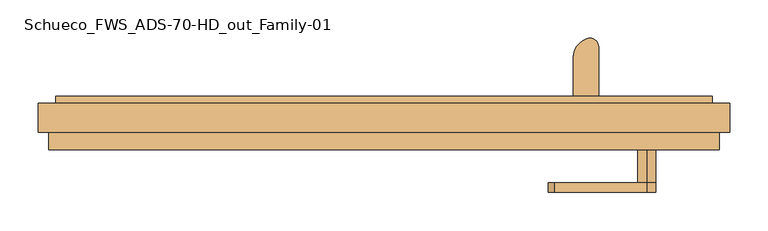
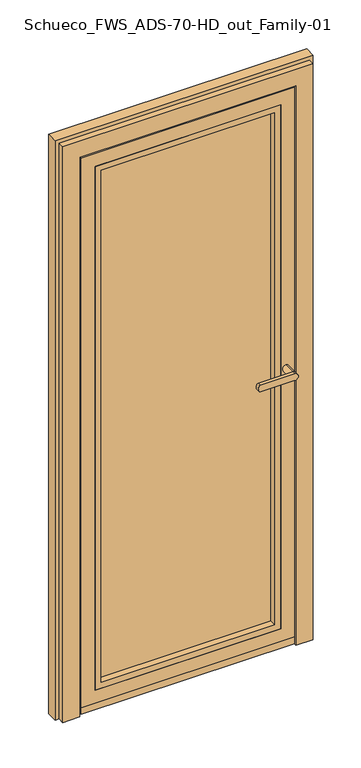
"""IFC4 building model written with IfcOpenShell, lengths in millimetres: door geometry, Schueco_FWS_ADS-70-HD_out_Family-01 : FWS SI insert unit."""

from ifc_helpers import new_model, si_unit, point, frame, frame_2d, origin, place, context, project, spatial, polyline, circle_curve, ellipse_curve, trimmed, segment, composite_curve, outline, extrude, faceted_brep, source, transform, mapped, element, save
from ifc_brep_helpers import plane_surface, cylinder_surface, extruded_surface, advanced_brep


def schueco_fws_ads_70_hd_out_family_01_db36a716(model_context):
    return source(origin(), model_context, "Body", "SolidModel", [
        extrude(outline(composite_curve([segment(polyline([(248.3337564, 8.9997177), (248.3337564, 59.1618682)]), True, "CONTINUOUS"), segment(trimmed(circle_curve(frame_2d((275.512174, 59.1618682)), 27.1784177), [point((248.3337564, 59.1618682))], [point((265.9750784, 84.6120194))], False, "CARTESIAN"), True, "CONTINUOUS"), segment(trimmed(circle_curve(frame_2d((270.0525794, 73.7310321)), 11.6198924), [point((265.9750784, 84.6120194))], [point((281.6724718, 73.7310321))], False, "CARTESIAN"), True, "CONTINUOUS"), segment(polyline([(281.6724718, 73.7310321), (281.6724718, 8.9997177), (248.3337564, 8.9997177)]), True, "CONTINUOUS")], self_intersect=False)), frame((0.0, 0.0, 2053.9218203), z_axis=(0.0, 0.0, 1.0), x_axis=(1.0, 0.0, 0.0)), (0.0, 0.0, 1.0), 4.0),
        extrude(outline(polyline([(248.3337564, 12.9997177), (281.6724718, 12.9997177), (281.6724718, 8.9997177), (248.3337564, 8.9997177), (248.3337564, 12.9997177)])), frame((0.0, 0.0, 2023.9218203), z_axis=(0.0, 0.0, 1.0), x_axis=(1.0, 0.0, 0.0)), (0.0, 0.0, 1.0), 30.0),
        extrude(outline(polyline([(248.3337564, 12.9997177), (281.6724718, 12.9997177), (281.6724718, 8.9997177), (248.3337564, 8.9997177), (248.3337564, 12.9997177)])), frame((0.0, 0.0, 49.9218203), z_axis=(0.0, 0.0, 1.0), x_axis=(1.0, 0.0, 0.0)), (0.0, 0.0, 1.0), 30.0),
        extrude(outline(composite_curve([segment(polyline([(248.3337564, 8.9997177), (248.3337564, 59.1618682)]), True, "CONTINUOUS"), segment(trimmed(circle_curve(frame_2d((275.512174, 59.1618682)), 27.1784177), [point((248.3337564, 59.1618682))], [point((265.9750784, 84.6120194))], False, "CARTESIAN"), True, "CONTINUOUS"), segment(trimmed(circle_curve(frame_2d((270.0525794, 73.7310321)), 11.6198924), [point((265.9750784, 84.6120194))], [point((281.6724718, 73.7310321))], False, "CARTESIAN"), True, "CONTINUOUS"), segment(polyline([(281.6724718, 73.7310321), (281.6724718, 8.9997177), (248.3337564, 8.9997177)]), True, "CONTINUOUS")], self_intersect=False)), frame((0.0, 0.0, 45.9218203), z_axis=(0.0, 0.0, 1.0), x_axis=(1.0, 0.0, 0.0)), (0.0, 0.0, 1.0), 4.0),
        advanced_brep(
        [(277.718156, 57.5977179, 2053.9218203), (252.2840039, 72.2821425, 2053.9218203), (277.718156, 57.5977179, 49.9218203), (252.2840039, 72.2821425, 49.9218203)],
        [
            (0, 1, ellipse_curve(frame((265.0010799, 64.9399302, 2053.9218203), z_axis=(0.0, 0.0, 1.0000000000000002), x_axis=(0.5000002582658958, 0.866025254674503, 0.0)), 21.5840887, 14.6844171)),
            (1, 0, ellipse_curve(frame((265.0010799, 64.9399302, 2053.9218203), z_axis=(0.0, 0.0, 1.0000000000000002), x_axis=(0.5000002582658958, 0.866025254674503, 0.0)), 21.5840887, 14.6844171)),
            (2, 3, ellipse_curve(frame((265.0010799, 64.9399302, 49.9218203), z_axis=(0.0, 0.0, -1.0000000000000002), x_axis=(-0.866025254674503, 0.5000002582658958, 0.0)), 14.6844171, 21.5840887)),
            (3, 2, ellipse_curve(frame((265.0010799, 64.9399302, 49.9218203), z_axis=(0.0, 0.0, -1.0000000000000002), x_axis=(-0.866025254674503, 0.5000002582658958, 0.0)), 14.6844171, 21.5840887)),
            (0, 2),
            (3, 1),
        ],
        [
            plane_surface(frame((252.2840039, 72.2821425, 2053.9218203), z_axis=(0.0, 0.0, 1.0000000000000002), x_axis=(0.5000002582658958, 0.866025254674503, 0.0))),
            plane_surface(frame((252.2840039, 72.2821425, 49.9218203), z_axis=(0.0, 0.0, -1.0000000000000002), x_axis=(-0.5000002582658958, -0.866025254674503, 0.0))),
            extruded_surface(trimmed(ellipse_curve(frame((265.0010799, 64.9399302, 49.9218203), z_axis=(0.0, 0.0, -1.0000000000000002), x_axis=(-0.866025254674503, 0.5000002582658958, 0.0)), 14.6844171, 21.5840887), [point((252.2840039, 72.2821425, 49.9218203))], [point((277.718156, 57.5977179, 49.9218203))], True, "CARTESIAN"), (0.0, 0.0, -2004.0), 2004.0),
            extruded_surface(trimmed(ellipse_curve(frame((265.0010799, 64.9399302, 49.9218203), z_axis=(0.0, 0.0, -1.0000000000000002), x_axis=(-0.866025254674503, 0.5000002582658958, 0.0)), 14.6844171, 21.5840887), [point((277.718156, 57.5977179, 49.9218203))], [point((252.2840039, 72.2821425, 49.9218203))], True, "CARTESIAN"), (0.0, 0.0, -2004.0), 2004.0),
        ],
        [
            (0, [[1, 2]]),
            (1, [[3, 4]]),
            (2, [[5, -4, 6, -1]]),
            (3, [[-6, -3, -5, -2]]),
        ],
    ),
        advanced_brep(
        [(345.0010799, -117.0002518, 1030.9991882), (345.0010799, -117.0002518, 1054.9764498), (223.3392873, -117.0002518, 1054.9764498), (223.3392873, -117.0002518, 1030.9991882), (345.0010799, -104.5001648, 1054.9764498), (345.0010799, -104.5001648, 1030.9991882), (223.3392873, -104.5001648, 1030.9991882), (223.3392873, -104.5001648, 1054.9764498), (345.0010799, -61.0002823, 1030.9991882), (345.0010799, -61.0002823, 1054.9764498)],
        [
            (0, 1, circle_curve(frame((345.0010799, -117.0002518, 1042.987819), z_axis=(0.0, -1.0, 0.0), x_axis=(0.0, 0.0, 1.0)), 11.9886308)),
            (1, 2),
            (2, 3, ellipse_curve(frame((223.3392873, -117.0002518, 1042.987819), z_axis=(0.0, -1.0, 0.0), x_axis=(0.0, 0.0, -1.0)), 11.9886308, 7.9050795)),
            (3, 0),
            (4, 5, circle_curve(frame((345.0010799, -104.5001648, 1042.987819), z_axis=(0.0, -1.0, 0.0), x_axis=(0.0, 0.0, 1.0)), 11.9886308)),
            (5, 6),
            (6, 7, ellipse_curve(frame((223.3392873, -104.5001648, 1042.987819), z_axis=(0.0, 1.0, 0.0), x_axis=(0.0, 0.0, -1.0)), 11.9886308, 7.9050795)),
            (7, 4),
            (3, 6),
            (5, 0),
            (2, 7),
            (1, 4),
            (5, 4, circle_curve(frame((345.0010799, -104.5001648, 1042.987819), z_axis=(0.0, -1.0, 0.0), x_axis=(0.0, 0.0, 1.0)), 11.9886308)),
            (8, 9, circle_curve(frame((345.0010799, -61.0002823, 1042.987819), z_axis=(0.0, 1.0, 0.0), x_axis=(0.0, 0.0, 1.0)), 11.9886308)),
            (9, 8, circle_curve(frame((345.0010799, -61.0002823, 1042.987819), z_axis=(0.0, 1.0, 0.0), x_axis=(0.0, 0.0, 1.0)), 11.9886308)),
            (8, 5),
            (4, 9),
        ],
        [
            plane_surface(frame((223.3392873, -117.0002518, 1030.9991882), z_axis=(0.0, -1.0, 0.0), x_axis=(-1.0, 0.0, 0.0))),
            plane_surface(frame((223.3392873, -104.5001648, 1030.9991882), z_axis=(0.0, 1.0, 0.0), x_axis=(1.0, 0.0, 0.0))),
            plane_surface(frame((345.0010799, -117.0002518, 1030.9991882), z_axis=(0.0, 0.0, -1.0), x_axis=(0.0, 1.0, 0.0))),
            extruded_surface(trimmed(ellipse_curve(frame((223.3392873, -104.5001648, 1042.987819), z_axis=(0.0, 1.0, 0.0), x_axis=(0.0, 0.0, -1.0)), 11.9886308, 7.9050795), [point((223.3392873, -104.5001648, 1030.9991882))], [point((223.3392873, -104.5001648, 1054.9764498))], True, "CARTESIAN"), (0.0, 12.500086999999994, 0.0), 12.500086999999994),
            plane_surface(frame((223.3392873, -117.0002518, 1054.9764498), z_axis=(0.0, 0.0, 1.0), x_axis=(0.0, 1.0, 0.0))),
            cylinder_surface(frame((345.0010799, -104.5001648, 1042.987819), z_axis=(0.0, -1.0, 0.0), x_axis=(0.0, 0.0, 1.0)), 11.9886308),
            plane_surface(frame((345.0010799, -61.0002823, 1054.9764498), z_axis=(0.0, 1.0, 0.0), x_axis=(-1.0, 0.0, 0.0))),
            cylinder_surface(frame((345.0010799, -61.0002823, 1042.987819), z_axis=(0.0, -1.0, 0.0), x_axis=(0.0, 0.0, 1.0)), 11.9886308),
        ],
        [
            (0, [[1, 2, 3, 4]]),
            (1, [[5, 6, 7, 8]]),
            (2, [[9, -6, 10, -4]]),
            (3, [[11, -7, -9, -3]]),
            (4, [[12, -8, -11, -2]]),
            (5, [[-10, 13, -12, -1]]),
            (6, [[14, 15]]),
            (7, [[16, -5, 17, -14]]),
            (7, [[-17, -13, -16, -15]]),
        ],
    ),
        extrude(outline(polyline([(80.9218203, 327.0670787), (2027.0538178, 327.0670787), (2027.0538178, -327.0649188), (80.9218203, -327.0649188), (80.9218203, 327.0670787)]), holes=[polyline([(102.9234681, -305.063271), (2005.05217, -305.063271), (2005.05217, 305.0654309), (102.9234681, 305.0654309), (102.9234681, -305.063271)])]), frame((0.0, -61.0002823, 0.0), z_axis=(0.0, 1.0, 0.0), x_axis=(0.0, 0.0, 1.0)), (0.0, 0.0, 1.0), 23.0002823),
        faceted_brep([(-375.0649188, -61.0002823, 2075.0538178), (-375.0649188, -52.5000065, 2075.0538178), (-375.0649188, -52.5000065, 32.9218203), (-375.0649188, -61.0002823, 32.9218203), (375.0670787, -52.5000065, 32.9218203), (375.0670787, -61.0002823, 32.9218203), (385.0670787, -52.5000065, 22.9218203), (385.0670787, -52.5000065, 2085.0538178), (-385.0649188, -52.5000065, 2085.0538178), (-385.0649188, -52.5000065, 22.9218203), (375.0670787, -52.5000065, 2075.0538178), (375.0670787, -61.0002823, 2075.0538178), (-327.0649188, -61.0002823, 80.9218203), (-327.0649188, -61.0002823, 2027.0538178), (327.0670787, -61.0002823, 2027.0538178), (327.0670787, -61.0002823, 80.9218203), (-327.0649188, 0.0, 2027.0538178), (-327.0649188, 0.0, 80.9218203), (327.0670787, 0.0, 80.9218203), (327.0670787, 0.0, 2027.0538178), (-302.0649188, 0.0, 105.9218203), (-302.0649188, 0.0, 2002.0538178), (302.0670787, 0.0, 2002.0538178), (302.0670787, 0.0, 105.9218203), (-302.0649188, 8.9997177, 2002.0538178), (-302.0649188, 8.9997177, 105.9218203), (302.0670787, 8.9997177, 105.9218203), (302.0670787, 8.9997177, 2002.0538178), (-400.0649188, 8.9997177, 7.9218203), (-400.0649188, 8.9997177, 2100.0538178), (400.0670787, 8.9997177, 2100.0538178), (400.0670787, 8.9997177, 7.9218203), (-400.0649188, 0.4997603, 2100.0538178), (-400.0649188, 0.4997603, 7.9218203), (400.0670787, 0.4997603, 7.9218203), (400.0670787, 0.4997603, 2100.0538178), (-385.0649188, 0.4997603, 22.9218203), (-385.0649188, 0.4997603, 2085.0538178), (385.0670787, 0.4997603, 2085.0538178), (385.0670787, 0.4997603, 22.9218203)], [[[0, 1, 2, 3]], [[3, 2, 4, 5]], [[6, 7, 8, 9], [2, 1, 10, 4]], [[5, 4, 10, 11]], [[5, 11, 0, 3], [12, 13, 14, 15]], [[16, 13, 12, 17]], [[17, 12, 15, 18]], [[18, 15, 14, 19]], [[18, 19, 16, 17], [20, 21, 22, 23]], [[24, 21, 20, 25]], [[25, 20, 23, 26]], [[26, 23, 22, 27]], [[28, 29, 30, 31], [26, 27, 24, 25]], [[32, 29, 28, 33]], [[33, 28, 31, 34]], [[34, 31, 30, 35]], [[34, 35, 32, 33], [36, 37, 38, 39]], [[8, 37, 36, 9]], [[9, 36, 39, 6]], [[6, 39, 38, 7]], [[11, 10, 1, 0]], [[19, 14, 13, 16]], [[27, 22, 21, 24]], [[35, 30, 29, 32]], [[7, 38, 37, 8]]]),
        extrude(outline(polyline([(327.0670787, -38.0), (-327.0649188, -38.0), (-327.0649188, 0.0), (327.0670787, 0.0), (327.0670787, -38.0)])), frame((0.0, 0.0, 80.9218203), z_axis=(0.0, 0.0, 1.0), x_axis=(1.0, 0.0, 0.0)), (0.0, 0.0, 1.0), 1946.1319975),
        extrude(outline(composite_curve([segment(polyline([(-26.4439202, 22.9218203), (-26.4439202, 4.2174554)]), True, "CONTINUOUS"), segment(trimmed(circle_curve(frame_2d((-37.0962864, 17.038728)), 16.6690713), [point((-26.4439202, 4.2174554))], [point((-47.7486527, 4.2174554))], False, "CARTESIAN"), True, "CONTINUOUS"), segment(polyline([(-47.7486527, 4.2174554), (-47.7486527, 22.9218203), (-26.4439202, 22.9218203)]), True, "CONTINUOUS")], self_intersect=False)), frame((-375.0649188, 0.0, 0.0), z_axis=(1.0, 0.0, 0.0), x_axis=(0.0, 1.0, 0.0)), (0.0, 0.0, 1.0), 750.1319975),
        extrude(outline(polyline([(-375.0649188, -61.0002823), (-375.0649188, -52.5000065), (375.0670787, -52.5000065), (375.0670787, -61.0002823), (-375.0649188, -61.0002823)])), frame((0.0, 0.0, 7.9218203), z_axis=(0.0, 0.0, 1.0), x_axis=(1.0, 0.0, 0.0)), (0.0, 0.0, 1.0), 25.0),
        faceted_brep([(430.999943, 8.9997177, 2130.999943), (430.999943, 0.0, 2130.999943), (430.999943, 0.0, 0.0), (430.999943, 8.9997177, 0.0), (-454.0, 0.0, 0.0), (-454.0, 0.0, 2154.0), (454.0, 0.0, 2154.0), (454.0, 0.0, 0.0), (-430.999943, 0.0, 2130.999943), (-430.999943, 0.0, 0.0), (454.0, -38.0, 0.0), (440.0, -38.0, 0.0), (440.0, -61.0002823, 0.0), (380.0652914, -61.0002823, 0.0), (380.0652914, -52.5000065, 0.0), (394.9999487, -52.5000065, 0.0), (394.9999487, 0.4997603, 0.0), (404.9999827, 0.4997603, 0.0), (404.9999827, 8.9997177, 0.0), (-404.9999827, 8.9997177, 0.0), (-430.999943, 8.9997177, 0.0), (-430.999943, 8.9997177, 2130.999943), (404.9999827, 8.9997177, 2104.9999827), (-404.9999827, 8.9997177, 2104.9999827), (380.0652914, -61.0002823, 2080.0652914), (380.0652914, -52.5000065, 2080.0652914), (-380.0652914, -52.5000065, 0.0), (-394.9999487, -52.5000065, 0.0), (-394.9999487, -52.5000065, 2094.9999487), (394.9999487, -52.5000065, 2094.9999487), (-380.0652914, -52.5000065, 2080.0652914), (-440.0, -61.0002823, 0.0), (-380.0652914, -61.0002823, 0.0), (-380.0652914, -61.0002823, 2080.0652914), (440.0, -61.0002823, 2140.0), (-440.0, -61.0002823, 2140.0), (440.0, -38.0, 2140.0), (-454.0, -38.0, 0.0), (-440.0, -38.0, 0.0), (-440.0, -38.0, 2140.0), (454.0, -38.0, 2154.0), (-454.0, -38.0, 2154.0), (-404.9999827, 0.4997603, 0.0), (-394.9999487, 0.4997603, 0.0), (404.9999827, 0.4997603, 2104.9999827), (-404.9999827, 0.4997603, 2104.9999827), (394.9999487, 0.4997603, 2094.9999487), (-394.9999487, 0.4997603, 2094.9999487)], [[[0, 1, 2, 3]], [[4, 5, 6, 7, 2, 1, 8, 9]], [[3, 2, 7, 10, 11, 12, 13, 14, 15, 16, 17, 18]], [[19, 20, 21, 0, 3, 18, 22, 23]], [[24, 25, 14, 13]], [[26, 27, 28, 29, 15, 14, 25, 30]], [[31, 32, 33, 24, 13, 12, 34, 35]], [[34, 12, 11, 36]], [[37, 38, 39, 36, 11, 10, 40, 41]], [[4, 9, 20, 19, 42, 43, 27, 26, 32, 31, 38, 37]], [[20, 9, 8, 21]], [[18, 17, 44, 22]], [[42, 19, 23, 45]], [[32, 26, 30, 33]], [[31, 35, 39, 38]], [[4, 37, 41, 5]], [[6, 40, 10, 7]], [[43, 42, 45, 44, 17, 16, 46, 47]], [[16, 15, 29, 46]], [[27, 43, 47, 28]], [[21, 8, 1, 0]], [[33, 30, 25, 24]], [[35, 34, 36, 39]], [[23, 22, 44, 45]], [[5, 41, 40, 6]], [[47, 46, 29, 28]]]),
    ])


if __name__ == "__main__":
    model = new_model("IFC4")
    model_context = context("Model", 3, world=origin())
    ifc_project = project(units=[si_unit("LENGTHUNIT", "METRE", prefix="MILLI")], contexts=[model_context])
    site = spatial("IfcSite", under=ifc_project)
    building = spatial("IfcBuilding", under=site)
    placement = place(None, origin())
    schueco_fws_ads_70_hd_out_family_01_shape = schueco_fws_ads_70_hd_out_family_01_db36a716(model_context)
    element("IfcDoor", 1, ObjectType="Schueco_FWS_ADS-70-HD_out_Family-01 : FWS SI insert unit", at=placement, inside=building, context=model_context, shape_type="MappedRepresentation", body=[
        mapped(schueco_fws_ads_70_hd_out_family_01_shape, transform((0.0, 0.0, 0.0), x_axis=(1.0, 0.0, 0.0), y_axis=(0.0, 1.0, 0.0), z_axis=(0.0, 0.0, 1.0))),
    ])
    save(model, "model.ifc")

# Revit data of these elements
# Type "Schueco_FWS_ADS-70-HD_out_Family-01 : FWS SI insert unit"
#   Type Mark = "44"
#   __NOTE__ = "Data describes the optimum values of the entire system. The properites of a selected design option have to be determined on an individual basis!"
#   Wind load resistance = "Class 2"
#   Watertightness = "Class 5A"
#   Thermal insulation = "Uf = 1.6 W/(m²K)"
#   Sound insulation = "to RW 43 db"
#   Schueco thermal insulation standard = "Thermally insulated"
#   Opening type = "Outward-opening, Flush-fitted"
#   Model = "Schueco ADS 70 HD"
#   Mechanical loading = "Class 2"
#   Maximum leaf width in mm = "1400"
#   Maximum leaf weight in kg = "200"
#   Maximum leaf height in mm = "3000"
#   Material = "Aluminium"
#   Construction Type = "Door, single-leaf, outward-opening"
#   Manufacturer = "Schueco International KG"
#   Long term functionality = "Class 6"
#   Glazing data = "Triple glazing 38mm"
#   Façade insert unit = "yes"
#   Family creation date = "08.2017"
#   Description = "Schueco Aluminium Door System (ADS)"
#   Burglar resistance = "Class RC 3"
#   Areas of use = "Public buildings"
#   Analytic Construction = "<None>"
#   Air permeability = "Class 2"
#   Width [instance default] = 624.636 mm
#   Leaf opening angle [instance default] = 0.00°
#   IOf_T = 38 mm
#   Height [instance default] = 1988.68 mm
#   Glazing area [instance default] = 0.554918 m²
#   Distance from bottom to handles [instance default] = 1050 mm
#   Clear opening width [instance default] = 476.636 mm
#   Standard threshold = no
#   Low level threshold = yes
#   Handles = yes
#   FWS SI insert unit = yes
#   FWS HI insert unit = no
#   Glass = none
#   Frame = Alu
#   Fittings = none
# Element 1 (IfcDoor, "Schueco_FWS_ADS-70-HD_out_Family-01 : FWS SI insert unit")
#   Width = 908 mm
#   Height = 2154 mm
#   Glazing area = 1.14518 m²
#   Clear opening width = 760 mm
#   Materials on its faces: "Alu", "Glass"
# Materials
#   "Alu": class "Glas", colour RGB 140 140 140, transparency 0
#   "Glass": class "Glass", colour RGB 128 128 255, transparency 0.75, Description = "Soda Lime Glass", Cost = 0
